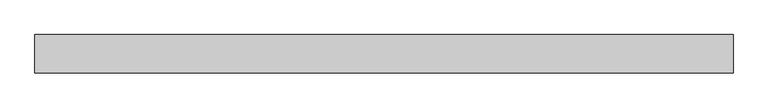
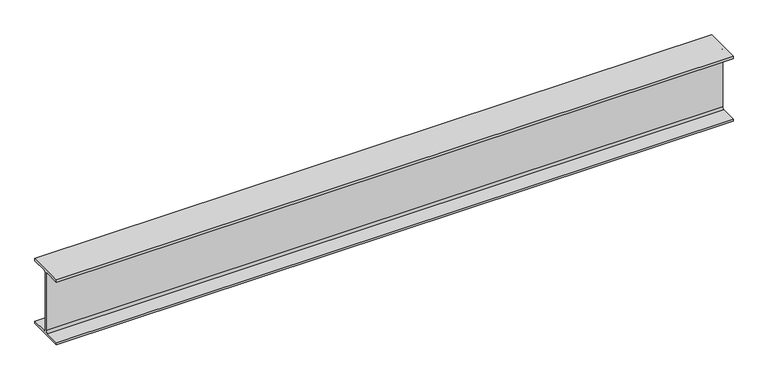
"""IFC4 building model written with IfcOpenShell, lengths in millimetres: beam geometry, Old_Steel Beam_H-KSD3502 : H_SB_ASB_H-250×125x6x9."""

from ifc_helpers import new_model, si_unit, point, frame, frame_2d, origin, place, context, project, spatial, polyline, circle_curve, trimmed, segment, composite_curve, outline, extrude, source, transform, mapped, element, save


def beam_841f7af1(model_context):
    return source(origin(), model_context, "Body", "SweptSolid", [
        extrude(outline(composite_curve([segment(polyline([(82.5, -141.5), (82.5, -151.7), (-82.5, -151.7), (-82.5, -141.5), (-11.9, -141.5)]), True, "CONTINUOUS"), segment(trimmed(circle_curve(frame_2d((-11.9, -132.6)), 8.9), [point((-11.9, -141.5))], [point((-3.0, -132.6))], True, "CARTESIAN"), True, "CONTINUOUS"), segment(polyline([(-3.0, -132.6), (-3.0, 132.6)]), True, "CONTINUOUS"), segment(trimmed(circle_curve(frame_2d((-11.9, 132.6)), 8.9), [point((-3.0, 132.6))], [point((-11.9, 141.5))], True, "CARTESIAN"), True, "CONTINUOUS"), segment(polyline([(-11.9, 141.5), (-82.5, 141.5), (-82.5, 151.7), (82.5, 151.7), (82.5, 141.5), (11.9, 141.5)]), True, "CONTINUOUS"), segment(trimmed(circle_curve(frame_2d((11.9, 132.6)), 8.9), [point((11.9, 141.5))], [point((3.0, 132.6))], True, "CARTESIAN"), True, "CONTINUOUS"), segment(polyline([(3.0, 132.6), (3.0, -132.6)]), True, "CONTINUOUS"), segment(trimmed(circle_curve(frame_2d((11.9, -132.6)), 8.9), [point((3.0, -132.6))], [point((11.9, -141.5))], True, "CARTESIAN"), True, "CONTINUOUS"), segment(polyline([(11.9, -141.5), (82.5, -141.5)]), True, "CONTINUOUS")], self_intersect=False)), frame((-1493.3, 0.0, 0.0), z_axis=(1.0, 0.0, 0.0), x_axis=(0.0, 1.0, 0.0)), (0.0, 0.0, 1.0), 2987.8360727),
    ])


if __name__ == "__main__":
    model = new_model("IFC4")
    model_context = context("Model", 3, world=origin())
    ifc_project = project(units=[si_unit("LENGTHUNIT", "METRE", prefix="MILLI")], contexts=[model_context])
    site = spatial("IfcSite", under=ifc_project)
    building = spatial("IfcBuilding", under=site)
    placement = place(None, origin())
    beam_shape = beam_841f7af1(model_context)
    element("IfcBeam", 1, ObjectType="Old_Steel Beam_H-KSD3502 : H_SB_ASB_H-250×125x6x9", at=placement, inside=building, context=model_context, shape_type="MappedRepresentation", body=[
        mapped(beam_shape, transform((0.0, 0.0, 0.0), x_axis=(1.0, 0.0, 0.0), y_axis=(0.0, 1.0, 0.0), z_axis=(0.0, 0.0, 1.0))),
    ])
    save(model, "model.ifc")

# Revit data of these elements
# Type "Old_Steel Beam_H-KSD3502 : H_SB_ASB_H-250×125x6x9"
#   Width = 12.5 cm
#   Web Thickness = 0.6 cm
#   Web Fillet = 1.2 cm
#   Warping Constant = 42539.8 cm⁶
#   Torsional Moment of Inertia = 7.8102 cm⁴
#   Torsional Modulus = 1.0 cm³
#   Section Area = 37.66 cm²
#   Plastic Modulus weak axis = 73.1 cm³
#   Plastic Modulus strong axis = 366.0 cm³
#   Perimeter = 0.97 m²/m
#   Nominal Weight = 29.60 kgf/m
#   Moment of Inertia weak axis = 294.00 cm⁴
#   Moment of Inertia strong axis = 4050.00 cm⁴
#   Height = 25.0 cm
#   Flange Thickness = 0.9 cm
#   Elastic Modulus weak axis = 47.0 cm³
#   Elastic Modulus strong axis = 324.0 cm³
#   Centroid Vertical = 12.5 cm
#   Centroid Horizontal = 6.25 cm
#   Length [instance default] = 1.5240 m
#   Structural Material [instance default] = Steel, 45-345
#   Assembly Code = ""
# Element 1 (IfcBeam, "Old_Steel Beam_H-KSD3502 : H_SB_ASB_H-250×125x6x9")
#   Structural Material = none
# Materials
#   "Steel, 45-345": class "Metal", colour RGB 189 187 185, transparency 0, Description = "Steel 345 MPa", Cost = 0
